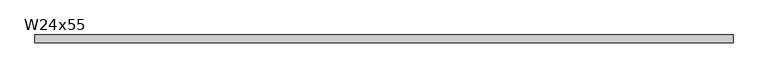
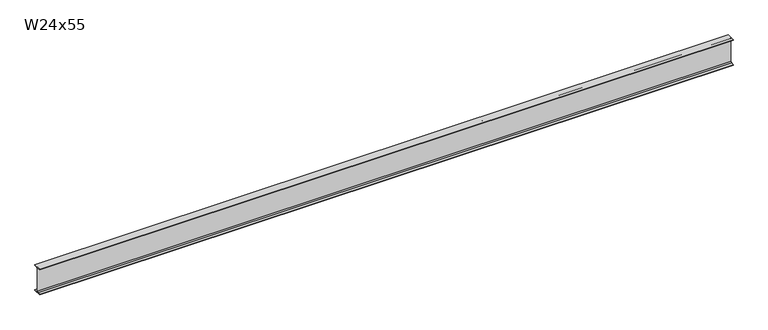
"""IFC4 building model written with IfcOpenShell, lengths in millimetres: beam geometry, RME W-Wide Flange : W24x55."""

from ifc_helpers import new_model, si_unit, point, frame, frame_2d, origin, place, context, project, spatial, polyline, circle_curve, trimmed, segment, composite_curve, outline, extrude, source, transform, mapped, element, save


def w24x55_4f807725(model_context):
    return source(origin(), model_context, "Body", "SweptSolid", [
        extrude(outline(composite_curve([segment(polyline([(89.027, -286.893), (89.027, -299.72), (-89.027, -299.72), (-89.027, -286.893), (-28.702, -286.893)]), True, "CONTINUOUS"), segment(trimmed(circle_curve(frame_2d((-28.702, -263.2075)), 23.6855), [point((-28.702, -286.893))], [point((-5.0165, -263.2075))], True, "CARTESIAN"), True, "CONTINUOUS"), segment(polyline([(-5.0165, -263.2075), (-5.0165, 263.2075)]), True, "CONTINUOUS"), segment(trimmed(circle_curve(frame_2d((-28.702, 263.2075)), 23.6855), [point((-5.0165, 263.2075))], [point((-28.702, 286.893))], True, "CARTESIAN"), True, "CONTINUOUS"), segment(polyline([(-28.702, 286.893), (-89.027, 286.893), (-89.027, 299.72), (89.027, 299.72), (89.027, 286.893), (28.702, 286.893)]), True, "CONTINUOUS"), segment(trimmed(circle_curve(frame_2d((28.702, 263.2075)), 23.6855), [point((28.702, 286.893))], [point((5.0165, 263.2075))], True, "CARTESIAN"), True, "CONTINUOUS"), segment(polyline([(5.0165, 263.2075), (5.0165, -263.2075)]), True, "CONTINUOUS"), segment(trimmed(circle_curve(frame_2d((28.702, -263.2075)), 23.6855), [point((5.0165, -263.2075))], [point((28.702, -286.893))], True, "CARTESIAN"), True, "CONTINUOUS"), segment(polyline([(28.702, -286.893), (89.027, -286.893)]), True, "CONTINUOUS")], self_intersect=False)), frame((-7642.6651201, 0.0, 0.0), z_axis=(1.0, 0.0, 0.0), x_axis=(0.0, 1.0, 0.0)), (0.0, 0.0, 1.0), 15392.8786531),
    ])


if __name__ == "__main__":
    model = new_model("IFC4")
    model_context = context("Model", 3, world=origin())
    ifc_project = project(units=[si_unit("LENGTHUNIT", "METRE", prefix="MILLI")], contexts=[model_context])
    site = spatial("IfcSite", under=ifc_project)
    building = spatial("IfcBuilding", under=site)
    placement = place(None, origin())
    w24x55_shape = w24x55_4f807725(model_context)
    element("IfcBeam", 1, ObjectType="RME W-Wide Flange : W24x55", at=placement, inside=building, context=model_context, shape_type="MappedRepresentation", body=[
        mapped(w24x55_shape, transform((0.0, 0.0, 0.0), x_axis=(1.0, 0.0, 0.0), y_axis=(0.0, 1.0, 0.0), z_axis=(0.0, 0.0, 1.0))),
    ])
    save(model, "model.ifc")

# Revit data of these elements
# Type "RME W-Wide Flange : W24x55"
#   WELD P [instance default] = ""
#   WELD LE [instance default] = ""
#   WELD D [instance default] = ""
#   TOP SECTION SIZE [instance default] = ""
#   TOP SECTION LENGTH [instance default] = ""
#   REMARKS [instance default] = ""
#   REINF TYPE [instance default] = ""
#   Nominal Size = "W24"
#   End Bearing Capacity [instance default] = ""
#   BOT SECTION SIZE [instance default] = ""
#   BOT SECTION LENGTH [instance default] = ""
#   Assembly Code = "B10"
#   W = 55
#   Start Extension Calculation [instance default] = 10' - 0"
#   Start Extension [instance default] = -0' - 0 1/2"
#   End Extension Calculation [instance default] = 10' - 0"
#   End Extension [instance default] = -0' - 0 1/2"
#   Length [instance default] = 5' - 0"
#   bf = 0' - 7.01"
#   d = 1' - 11.6"
#   k = 0' - 1 7/16"
#   k2 = 0' - 0.9325"
#   tf = 0' - 0.505"
#   tw = 0' - 0.395"
#   A = 0.1125 SF
#   Structural Material [instance default] = Metal - Steel - ASTM A992
# Element 1 (IfcBeam, "RME W-Wide Flange : W24x55")
#   Length = 50' - 10.25303"
#   Materials on its faces: "Metal - Steel - ASTM A992"
# Materials
#   "Metal - Steel - ASTM A992": class "Metal", colour RGB 255 128 0, transparency 0
